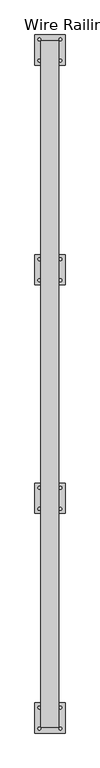
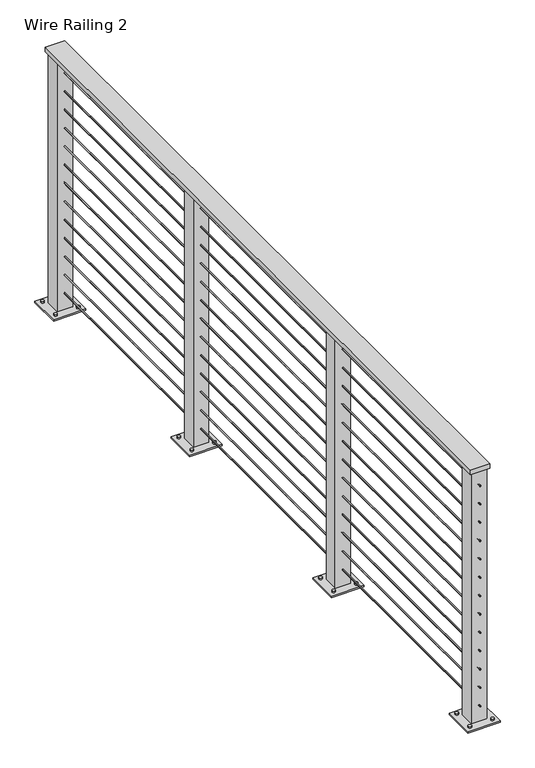
"""IFC4 building model written with IfcOpenShell, lengths in millimetres: railing geometry, Wire Railing 2."""

from ifc_helpers import new_model, si_unit, point, frame, frame_2d, origin, place, context, project, spatial, polyline, circle_curve, trimmed, segment, composite_curve, outline, extrude, source, transform, mapped, element, save


def wire_railing_2_0188c66e(model_context):
    return source(origin(), model_context, "Body", "SweptSolid", [
        extrude(outline(polyline([(25886.5620052, 5898.8634079), (25962.7620052, 5898.8634079), (25962.7620052, 3003.2634079), (25886.5620052, 3003.2634079), (25886.5620052, 5898.8634079)])), frame((0.0, 0.0, 3851.275), z_axis=(0.0, 0.0, 1.0), x_axis=(1.0, 0.0, 0.0)), (0.0, 0.0, 1.0), 19.05),
        extrude(outline(composite_curve([segment(trimmed(circle_curve(frame_2d((3791.74375, 25924.6620052)), 2.38125), [point((3791.74375, 25927.0432552))], [point((3791.74375, 25922.2807552))], False, "CARTESIAN"), True, "CONTINUOUS"), segment(trimmed(circle_curve(frame_2d((3791.74375, 25924.6620052)), 2.38125), [point((3791.74375, 25922.2807552))], [point((3791.74375, 25927.0432552))], False, "CARTESIAN"), True, "CONTINUOUS")], self_intersect=False)), frame((0.0, 3003.2634079, 0.0), z_axis=(0.0, 1.0, 0.0), x_axis=(0.0, 0.0, 1.0)), (0.0, 0.0, 1.0), 2895.6),
        extrude(outline(composite_curve([segment(trimmed(circle_curve(frame_2d((3715.54375, 25924.6620052)), 2.38125), [point((3715.54375, 25927.0432552))], [point((3715.54375, 25922.2807552))], False, "CARTESIAN"), True, "CONTINUOUS"), segment(trimmed(circle_curve(frame_2d((3715.54375, 25924.6620052)), 2.38125), [point((3715.54375, 25922.2807552))], [point((3715.54375, 25927.0432552))], False, "CARTESIAN"), True, "CONTINUOUS")], self_intersect=False)), frame((0.0, 3003.2634079, 0.0), z_axis=(0.0, 1.0, 0.0), x_axis=(0.0, 0.0, 1.0)), (0.0, 0.0, 1.0), 2895.6),
        extrude(outline(composite_curve([segment(trimmed(circle_curve(frame_2d((3639.34375, 25924.6620052)), 2.38125), [point((3639.34375, 25927.0432552))], [point((3639.34375, 25922.2807552))], False, "CARTESIAN"), True, "CONTINUOUS"), segment(trimmed(circle_curve(frame_2d((3639.34375, 25924.6620052)), 2.38125), [point((3639.34375, 25922.2807552))], [point((3639.34375, 25927.0432552))], False, "CARTESIAN"), True, "CONTINUOUS")], self_intersect=False)), frame((0.0, 3003.2634079, 0.0), z_axis=(0.0, 1.0, 0.0), x_axis=(0.0, 0.0, 1.0)), (0.0, 0.0, 1.0), 2895.6),
        extrude(outline(composite_curve([segment(trimmed(circle_curve(frame_2d((3563.14375, 25924.6620052)), 2.38125), [point((3563.14375, 25927.0432552))], [point((3563.14375, 25922.2807552))], False, "CARTESIAN"), True, "CONTINUOUS"), segment(trimmed(circle_curve(frame_2d((3563.14375, 25924.6620052)), 2.38125), [point((3563.14375, 25922.2807552))], [point((3563.14375, 25927.0432552))], False, "CARTESIAN"), True, "CONTINUOUS")], self_intersect=False)), frame((0.0, 3003.2634079, 0.0), z_axis=(0.0, 1.0, 0.0), x_axis=(0.0, 0.0, 1.0)), (0.0, 0.0, 1.0), 2895.6),
        extrude(outline(composite_curve([segment(trimmed(circle_curve(frame_2d((3486.94375, 25924.6620052)), 2.38125), [point((3486.94375, 25927.0432552))], [point((3486.94375, 25922.2807552))], False, "CARTESIAN"), True, "CONTINUOUS"), segment(trimmed(circle_curve(frame_2d((3486.94375, 25924.6620052)), 2.38125), [point((3486.94375, 25922.2807552))], [point((3486.94375, 25927.0432552))], False, "CARTESIAN"), True, "CONTINUOUS")], self_intersect=False)), frame((0.0, 3003.2634079, 0.0), z_axis=(0.0, 1.0, 0.0), x_axis=(0.0, 0.0, 1.0)), (0.0, 0.0, 1.0), 2895.6),
        extrude(outline(composite_curve([segment(trimmed(circle_curve(frame_2d((3410.74375, 25924.6620052)), 2.38125), [point((3410.74375, 25927.0432552))], [point((3410.74375, 25922.2807552))], False, "CARTESIAN"), True, "CONTINUOUS"), segment(trimmed(circle_curve(frame_2d((3410.74375, 25924.6620052)), 2.38125), [point((3410.74375, 25922.2807552))], [point((3410.74375, 25927.0432552))], False, "CARTESIAN"), True, "CONTINUOUS")], self_intersect=False)), frame((0.0, 3003.2634079, 0.0), z_axis=(0.0, 1.0, 0.0), x_axis=(0.0, 0.0, 1.0)), (0.0, 0.0, 1.0), 2895.6),
        extrude(outline(composite_curve([segment(trimmed(circle_curve(frame_2d((3334.54375, 25924.6620052)), 2.38125), [point((3334.54375, 25927.0432552))], [point((3334.54375, 25922.2807552))], False, "CARTESIAN"), True, "CONTINUOUS"), segment(trimmed(circle_curve(frame_2d((3334.54375, 25924.6620052)), 2.38125), [point((3334.54375, 25922.2807552))], [point((3334.54375, 25927.0432552))], False, "CARTESIAN"), True, "CONTINUOUS")], self_intersect=False)), frame((0.0, 3003.2634079, 0.0), z_axis=(0.0, 1.0, 0.0), x_axis=(0.0, 0.0, 1.0)), (0.0, 0.0, 1.0), 2895.6),
        extrude(outline(composite_curve([segment(trimmed(circle_curve(frame_2d((3258.34375, 25924.6620052)), 2.38125), [point((3258.34375, 25927.0432552))], [point((3258.34375, 25922.2807552))], False, "CARTESIAN"), True, "CONTINUOUS"), segment(trimmed(circle_curve(frame_2d((3258.34375, 25924.6620052)), 2.38125), [point((3258.34375, 25922.2807552))], [point((3258.34375, 25927.0432552))], False, "CARTESIAN"), True, "CONTINUOUS")], self_intersect=False)), frame((0.0, 3003.2634079, 0.0), z_axis=(0.0, 1.0, 0.0), x_axis=(0.0, 0.0, 1.0)), (0.0, 0.0, 1.0), 2895.6),
        extrude(outline(composite_curve([segment(trimmed(circle_curve(frame_2d((3182.14375, 25924.6620052)), 2.38125), [point((3182.14375, 25927.0432552))], [point((3182.14375, 25922.2807552))], False, "CARTESIAN"), True, "CONTINUOUS"), segment(trimmed(circle_curve(frame_2d((3182.14375, 25924.6620052)), 2.38125), [point((3182.14375, 25922.2807552))], [point((3182.14375, 25927.0432552))], False, "CARTESIAN"), True, "CONTINUOUS")], self_intersect=False)), frame((0.0, 3003.2634079, 0.0), z_axis=(0.0, 1.0, 0.0), x_axis=(0.0, 0.0, 1.0)), (0.0, 0.0, 1.0), 2895.6),
        extrude(outline(composite_curve([segment(trimmed(circle_curve(frame_2d((3105.94375, 25924.6620052)), 2.38125), [point((3105.94375, 25927.0432552))], [point((3105.94375, 25922.2807552))], False, "CARTESIAN"), True, "CONTINUOUS"), segment(trimmed(circle_curve(frame_2d((3105.94375, 25924.6620052)), 2.38125), [point((3105.94375, 25922.2807552))], [point((3105.94375, 25927.0432552))], False, "CARTESIAN"), True, "CONTINUOUS")], self_intersect=False)), frame((0.0, 3003.2634079, 0.0), z_axis=(0.0, 1.0, 0.0), x_axis=(0.0, 0.0, 1.0)), (0.0, 0.0, 1.0), 2895.6),
        extrude(outline(composite_curve([segment(trimmed(circle_curve(frame_2d((3029.74375, 25924.6620052)), 2.38125), [point((3029.74375, 25927.0432552))], [point((3029.74375, 25922.2807552))], False, "CARTESIAN"), True, "CONTINUOUS"), segment(trimmed(circle_curve(frame_2d((3029.74375, 25924.6620052)), 2.38125), [point((3029.74375, 25922.2807552))], [point((3029.74375, 25927.0432552))], False, "CARTESIAN"), True, "CONTINUOUS")], self_intersect=False)), frame((0.0, 3003.2634079, 0.0), z_axis=(0.0, 1.0, 0.0), x_axis=(0.0, 0.0, 1.0)), (0.0, 0.0, 1.0), 2895.6),
        extrude(outline(composite_curve([segment(trimmed(circle_curve(frame_2d((2953.54375, 25924.6620052)), 2.38125), [point((2953.54375, 25927.0432552))], [point((2953.54375, 25922.2807552))], False, "CARTESIAN"), True, "CONTINUOUS"), segment(trimmed(circle_curve(frame_2d((2953.54375, 25924.6620052)), 2.38125), [point((2953.54375, 25922.2807552))], [point((2953.54375, 25927.0432552))], False, "CARTESIAN"), True, "CONTINUOUS")], self_intersect=False)), frame((0.0, 3003.2634079, 0.0), z_axis=(0.0, 1.0, 0.0), x_axis=(0.0, 0.0, 1.0)), (0.0, 0.0, 1.0), 2895.6),
        extrude(outline(composite_curve([segment(trimmed(circle_curve(frame_2d((2877.34375, 25924.6620052)), 2.38125), [point((2877.34375, 25927.0432552))], [point((2877.34375, 25922.2807552))], False, "CARTESIAN"), True, "CONTINUOUS"), segment(trimmed(circle_curve(frame_2d((2877.34375, 25924.6620052)), 2.38125), [point((2877.34375, 25922.2807552))], [point((2877.34375, 25927.0432552))], False, "CARTESIAN"), True, "CONTINUOUS")], self_intersect=False)), frame((0.0, 3003.2634079, 0.0), z_axis=(0.0, 1.0, 0.0), x_axis=(0.0, 0.0, 1.0)), (0.0, 0.0, 1.0), 2895.6),
        extrude(outline(composite_curve([segment(trimmed(circle_curve(frame_2d((25880.2120052, 4012.9134079)), 6.35), [point((25873.8620052, 4012.9134079))], [point((25886.5620052, 4012.9134079))], False, "CARTESIAN"), True, "CONTINUOUS"), segment(trimmed(circle_curve(frame_2d((25880.2120052, 4012.9134079)), 6.35), [point((25886.5620052, 4012.9134079))], [point((25873.8620052, 4012.9134079))], False, "CARTESIAN"), True, "CONTINUOUS")], self_intersect=False)), frame((0.0, 0.0, 2803.525), z_axis=(0.0, 0.0, 1.0), x_axis=(1.0, 0.0, 0.0)), (0.0, 0.0, 1.0), 12.7),
        extrude(outline(composite_curve([segment(trimmed(circle_curve(frame_2d((25969.1120052, 4012.9134079)), 6.35), [point((25962.7620052, 4012.9134079))], [point((25975.4620052, 4012.9134079))], False, "CARTESIAN"), True, "CONTINUOUS"), segment(trimmed(circle_curve(frame_2d((25969.1120052, 4012.9134079)), 6.35), [point((25975.4620052, 4012.9134079))], [point((25962.7620052, 4012.9134079))], False, "CARTESIAN"), True, "CONTINUOUS")], self_intersect=False)), frame((0.0, 0.0, 2803.525), z_axis=(0.0, 0.0, 1.0), x_axis=(1.0, 0.0, 0.0)), (0.0, 0.0, 1.0), 12.7),
        extrude(outline(composite_curve([segment(trimmed(circle_curve(frame_2d((25880.2120052, 3924.0134079)), 6.35), [point((25873.8620052, 3924.0134079))], [point((25886.5620052, 3924.0134079))], False, "CARTESIAN"), True, "CONTINUOUS"), segment(trimmed(circle_curve(frame_2d((25880.2120052, 3924.0134079)), 6.35), [point((25886.5620052, 3924.0134079))], [point((25873.8620052, 3924.0134079))], False, "CARTESIAN"), True, "CONTINUOUS")], self_intersect=False)), frame((0.0, 0.0, 2803.525), z_axis=(0.0, 0.0, 1.0), x_axis=(1.0, 0.0, 0.0)), (0.0, 0.0, 1.0), 12.7),
        extrude(outline(composite_curve([segment(trimmed(circle_curve(frame_2d((25969.1120052, 3924.0134079)), 6.35), [point((25962.7620052, 3924.0134079))], [point((25975.4620052, 3924.0134079))], False, "CARTESIAN"), True, "CONTINUOUS"), segment(trimmed(circle_curve(frame_2d((25969.1120052, 3924.0134079)), 6.35), [point((25975.4620052, 3924.0134079))], [point((25962.7620052, 3924.0134079))], False, "CARTESIAN"), True, "CONTINUOUS")], self_intersect=False)), frame((0.0, 0.0, 2803.525), z_axis=(0.0, 0.0, 1.0), x_axis=(1.0, 0.0, 0.0)), (0.0, 0.0, 1.0), 12.7),
        extrude(outline(polyline([(25988.1620052, 4031.9634079), (25988.1620052, 3904.9634079), (25861.1620052, 3904.9634079), (25861.1620052, 4031.9634079), (25988.1620052, 4031.9634079)])), frame((0.0, 0.0, 2803.525), z_axis=(0.0, 0.0, 1.0), x_axis=(1.0, 0.0, 0.0)), (0.0, 0.0, 1.0), 6.35),
        extrude(outline(polyline([(25954.8245052, 3998.6259079), (25954.8245052, 3938.3009079), (25894.4995052, 3938.3009079), (25894.4995052, 3998.6259079), (25954.8245052, 3998.6259079)]), holes=[polyline([(25948.4745052, 3992.2759079), (25900.8495052, 3992.2759079), (25900.8495052, 3944.6509079), (25948.4745052, 3944.6509079), (25948.4745052, 3992.2759079)])]), frame((0.0, 0.0, 2803.525), z_axis=(0.0, 0.0, 1.0), x_axis=(1.0, 0.0, 0.0)), (0.0, 0.0, 1.0), 1047.75),
        extrude(outline(composite_curve([segment(trimmed(circle_curve(frame_2d((25880.2120052, 4978.1134079)), 6.35), [point((25873.8620052, 4978.1134079))], [point((25886.5620052, 4978.1134079))], False, "CARTESIAN"), True, "CONTINUOUS"), segment(trimmed(circle_curve(frame_2d((25880.2120052, 4978.1134079)), 6.35), [point((25886.5620052, 4978.1134079))], [point((25873.8620052, 4978.1134079))], False, "CARTESIAN"), True, "CONTINUOUS")], self_intersect=False)), frame((0.0, 0.0, 2803.525), z_axis=(0.0, 0.0, 1.0), x_axis=(1.0, 0.0, 0.0)), (0.0, 0.0, 1.0), 12.7),
        extrude(outline(composite_curve([segment(trimmed(circle_curve(frame_2d((25969.1120052, 4978.1134079)), 6.35), [point((25962.7620052, 4978.1134079))], [point((25975.4620052, 4978.1134079))], False, "CARTESIAN"), True, "CONTINUOUS"), segment(trimmed(circle_curve(frame_2d((25969.1120052, 4978.1134079)), 6.35), [point((25975.4620052, 4978.1134079))], [point((25962.7620052, 4978.1134079))], False, "CARTESIAN"), True, "CONTINUOUS")], self_intersect=False)), frame((0.0, 0.0, 2803.525), z_axis=(0.0, 0.0, 1.0), x_axis=(1.0, 0.0, 0.0)), (0.0, 0.0, 1.0), 12.7),
        extrude(outline(composite_curve([segment(trimmed(circle_curve(frame_2d((25880.2120052, 4889.2134079)), 6.35), [point((25873.8620052, 4889.2134079))], [point((25886.5620052, 4889.2134079))], False, "CARTESIAN"), True, "CONTINUOUS"), segment(trimmed(circle_curve(frame_2d((25880.2120052, 4889.2134079)), 6.35), [point((25886.5620052, 4889.2134079))], [point((25873.8620052, 4889.2134079))], False, "CARTESIAN"), True, "CONTINUOUS")], self_intersect=False)), frame((0.0, 0.0, 2803.525), z_axis=(0.0, 0.0, 1.0), x_axis=(1.0, 0.0, 0.0)), (0.0, 0.0, 1.0), 12.7),
        extrude(outline(composite_curve([segment(trimmed(circle_curve(frame_2d((25969.1120052, 4889.2134079)), 6.35), [point((25962.7620052, 4889.2134079))], [point((25975.4620052, 4889.2134079))], False, "CARTESIAN"), True, "CONTINUOUS"), segment(trimmed(circle_curve(frame_2d((25969.1120052, 4889.2134079)), 6.35), [point((25975.4620052, 4889.2134079))], [point((25962.7620052, 4889.2134079))], False, "CARTESIAN"), True, "CONTINUOUS")], self_intersect=False)), frame((0.0, 0.0, 2803.525), z_axis=(0.0, 0.0, 1.0), x_axis=(1.0, 0.0, 0.0)), (0.0, 0.0, 1.0), 12.7),
        extrude(outline(polyline([(25988.1620052, 4997.1634079), (25988.1620052, 4870.1634079), (25861.1620052, 4870.1634079), (25861.1620052, 4997.1634079), (25988.1620052, 4997.1634079)])), frame((0.0, 0.0, 2803.525), z_axis=(0.0, 0.0, 1.0), x_axis=(1.0, 0.0, 0.0)), (0.0, 0.0, 1.0), 6.35),
        extrude(outline(polyline([(25954.8245052, 4963.8259079), (25954.8245052, 4903.5009079), (25894.4995052, 4903.5009079), (25894.4995052, 4963.8259079), (25954.8245052, 4963.8259079)]), holes=[polyline([(25948.4745052, 4957.4759079), (25900.8495052, 4957.4759079), (25900.8495052, 4909.8509079), (25948.4745052, 4909.8509079), (25948.4745052, 4957.4759079)])]), frame((0.0, 0.0, 2803.525), z_axis=(0.0, 0.0, 1.0), x_axis=(1.0, 0.0, 0.0)), (0.0, 0.0, 1.0), 1047.75),
        extrude(outline(composite_curve([segment(trimmed(circle_curve(frame_2d((25880.2120052, 3085.8134079)), 6.35), [point((25873.8620052, 3085.8134079))], [point((25886.5620052, 3085.8134079))], False, "CARTESIAN"), True, "CONTINUOUS"), segment(trimmed(circle_curve(frame_2d((25880.2120052, 3085.8134079)), 6.35), [point((25886.5620052, 3085.8134079))], [point((25873.8620052, 3085.8134079))], False, "CARTESIAN"), True, "CONTINUOUS")], self_intersect=False)), frame((0.0, 0.0, 2803.525), z_axis=(0.0, 0.0, 1.0), x_axis=(1.0, 0.0, 0.0)), (0.0, 0.0, 1.0), 12.7),
        extrude(outline(composite_curve([segment(trimmed(circle_curve(frame_2d((25969.1120052, 3085.8134079)), 6.35), [point((25962.7620052, 3085.8134079))], [point((25975.4620052, 3085.8134079))], False, "CARTESIAN"), True, "CONTINUOUS"), segment(trimmed(circle_curve(frame_2d((25969.1120052, 3085.8134079)), 6.35), [point((25975.4620052, 3085.8134079))], [point((25962.7620052, 3085.8134079))], False, "CARTESIAN"), True, "CONTINUOUS")], self_intersect=False)), frame((0.0, 0.0, 2803.525), z_axis=(0.0, 0.0, 1.0), x_axis=(1.0, 0.0, 0.0)), (0.0, 0.0, 1.0), 12.7),
        extrude(outline(composite_curve([segment(trimmed(circle_curve(frame_2d((25880.2120052, 2996.9134079)), 6.35), [point((25873.8620052, 2996.9134079))], [point((25886.5620052, 2996.9134079))], False, "CARTESIAN"), True, "CONTINUOUS"), segment(trimmed(circle_curve(frame_2d((25880.2120052, 2996.9134079)), 6.35), [point((25886.5620052, 2996.9134079))], [point((25873.8620052, 2996.9134079))], False, "CARTESIAN"), True, "CONTINUOUS")], self_intersect=False)), frame((0.0, 0.0, 2803.525), z_axis=(0.0, 0.0, 1.0), x_axis=(1.0, 0.0, 0.0)), (0.0, 0.0, 1.0), 12.7),
        extrude(outline(composite_curve([segment(trimmed(circle_curve(frame_2d((25969.1120052, 2996.9134079)), 6.35), [point((25962.7620052, 2996.9134079))], [point((25975.4620052, 2996.9134079))], False, "CARTESIAN"), True, "CONTINUOUS"), segment(trimmed(circle_curve(frame_2d((25969.1120052, 2996.9134079)), 6.35), [point((25975.4620052, 2996.9134079))], [point((25962.7620052, 2996.9134079))], False, "CARTESIAN"), True, "CONTINUOUS")], self_intersect=False)), frame((0.0, 0.0, 2803.525), z_axis=(0.0, 0.0, 1.0), x_axis=(1.0, 0.0, 0.0)), (0.0, 0.0, 1.0), 12.7),
        extrude(outline(polyline([(25988.1620052, 3104.8634079), (25988.1620052, 2977.8634079), (25861.1620052, 2977.8634079), (25861.1620052, 3104.8634079), (25988.1620052, 3104.8634079)])), frame((0.0, 0.0, 2803.525), z_axis=(0.0, 0.0, 1.0), x_axis=(1.0, 0.0, 0.0)), (0.0, 0.0, 1.0), 6.35),
        extrude(outline(polyline([(25954.8245052, 3071.5259079), (25954.8245052, 3011.2009079), (25894.4995052, 3011.2009079), (25894.4995052, 3071.5259079), (25954.8245052, 3071.5259079)]), holes=[polyline([(25948.4745052, 3065.1759079), (25900.8495052, 3065.1759079), (25900.8495052, 3017.5509079), (25948.4745052, 3017.5509079), (25948.4745052, 3065.1759079)])]), frame((0.0, 0.0, 2803.525), z_axis=(0.0, 0.0, 1.0), x_axis=(1.0, 0.0, 0.0)), (0.0, 0.0, 1.0), 1047.75),
        extrude(outline(composite_curve([segment(trimmed(circle_curve(frame_2d((25880.2120052, 5905.2134079)), 6.35), [point((25873.8620052, 5905.2134079))], [point((25886.5620052, 5905.2134079))], False, "CARTESIAN"), True, "CONTINUOUS"), segment(trimmed(circle_curve(frame_2d((25880.2120052, 5905.2134079)), 6.35), [point((25886.5620052, 5905.2134079))], [point((25873.8620052, 5905.2134079))], False, "CARTESIAN"), True, "CONTINUOUS")], self_intersect=False)), frame((0.0, 0.0, 2803.525), z_axis=(0.0, 0.0, 1.0), x_axis=(1.0, 0.0, 0.0)), (0.0, 0.0, 1.0), 12.7),
        extrude(outline(composite_curve([segment(trimmed(circle_curve(frame_2d((25969.1120052, 5905.2134079)), 6.35), [point((25962.7620052, 5905.2134079))], [point((25975.4620052, 5905.2134079))], False, "CARTESIAN"), True, "CONTINUOUS"), segment(trimmed(circle_curve(frame_2d((25969.1120052, 5905.2134079)), 6.35), [point((25975.4620052, 5905.2134079))], [point((25962.7620052, 5905.2134079))], False, "CARTESIAN"), True, "CONTINUOUS")], self_intersect=False)), frame((0.0, 0.0, 2803.525), z_axis=(0.0, 0.0, 1.0), x_axis=(1.0, 0.0, 0.0)), (0.0, 0.0, 1.0), 12.7),
        extrude(outline(composite_curve([segment(trimmed(circle_curve(frame_2d((25880.2120052, 5816.3134079)), 6.35), [point((25873.8620052, 5816.3134079))], [point((25886.5620052, 5816.3134079))], False, "CARTESIAN"), True, "CONTINUOUS"), segment(trimmed(circle_curve(frame_2d((25880.2120052, 5816.3134079)), 6.35), [point((25886.5620052, 5816.3134079))], [point((25873.8620052, 5816.3134079))], False, "CARTESIAN"), True, "CONTINUOUS")], self_intersect=False)), frame((0.0, 0.0, 2803.525), z_axis=(0.0, 0.0, 1.0), x_axis=(1.0, 0.0, 0.0)), (0.0, 0.0, 1.0), 12.7),
        extrude(outline(composite_curve([segment(trimmed(circle_curve(frame_2d((25969.1120052, 5816.3134079)), 6.35), [point((25962.7620052, 5816.3134079))], [point((25975.4620052, 5816.3134079))], False, "CARTESIAN"), True, "CONTINUOUS"), segment(trimmed(circle_curve(frame_2d((25969.1120052, 5816.3134079)), 6.35), [point((25975.4620052, 5816.3134079))], [point((25962.7620052, 5816.3134079))], False, "CARTESIAN"), True, "CONTINUOUS")], self_intersect=False)), frame((0.0, 0.0, 2803.525), z_axis=(0.0, 0.0, 1.0), x_axis=(1.0, 0.0, 0.0)), (0.0, 0.0, 1.0), 12.7),
        extrude(outline(polyline([(25988.1620052, 5924.2634079), (25988.1620052, 5797.2634079), (25861.1620052, 5797.2634079), (25861.1620052, 5924.2634079), (25988.1620052, 5924.2634079)])), frame((0.0, 0.0, 2803.525), z_axis=(0.0, 0.0, 1.0), x_axis=(1.0, 0.0, 0.0)), (0.0, 0.0, 1.0), 6.35),
        extrude(outline(polyline([(25954.8245052, 5890.9259079), (25954.8245052, 5830.6009079), (25894.4995052, 5830.6009079), (25894.4995052, 5890.9259079), (25954.8245052, 5890.9259079)]), holes=[polyline([(25948.4745052, 5884.5759079), (25900.8495052, 5884.5759079), (25900.8495052, 5836.9509079), (25948.4745052, 5836.9509079), (25948.4745052, 5884.5759079)])]), frame((0.0, 0.0, 2803.525), z_axis=(0.0, 0.0, 1.0), x_axis=(1.0, 0.0, 0.0)), (0.0, 0.0, 1.0), 1047.75),
    ])


if __name__ == "__main__":
    model = new_model("IFC4")
    model_context = context("Model", 3, world=origin())
    ifc_project = project(units=[si_unit("LENGTHUNIT", "METRE", prefix="MILLI")], contexts=[model_context])
    site = spatial("IfcSite", under=ifc_project)
    building = spatial("IfcBuilding", under=site)
    placement = place(None, origin())
    wire_railing_2_shape = wire_railing_2_0188c66e(model_context)
    element("IfcRailing", 1, ObjectType="Wire Railing 2", at=placement, inside=building, context=model_context, shape_type="MappedRepresentation", body=[
        mapped(wire_railing_2_shape, transform((0.0, 0.0, 0.0), x_axis=(1.0, 0.0, 0.0), y_axis=(0.0, 1.0, 0.0), z_axis=(0.0, 0.0, 1.0))),
    ])
    save(model, "model.ifc")

# Revit data of these elements
# Element 1 (IfcRailing, "Wire Railing 2")
#   Materials on its faces: "2 1/2\" X 2 1/2\" ALUM. SQUARE POST (38\" O.C. MAX)", "WIRE RAILING (3\" O.C.)", "ALUM. PLATE TOP RAIL"
# Materials
#   "2 1/2\" X 2 1/2\" ALUM. SQUARE POST (38\" O.C. MAX)": class "Metal", colour RGB 244 244 244, transparency 0, Manufacturer = "Kawneer", URL = "http://www.kawneer.com/kawneer/north_america/en/home.asp", Cost = 0
#   "WIRE RAILING (3\" O.C.)": class "Metal", colour RGB 244 244 244, transparency 0, Manufacturer = "Kawneer", URL = "http://www.kawneer.com/kawneer/north_america/en/home.asp", Cost = 0
#   "ALUM. PLATE TOP RAIL": class "Metal", colour RGB 244 244 244, transparency 0, Manufacturer = "Kawneer", URL = "http://www.kawneer.com/kawneer/north_america/en/home.asp", Cost = 0
